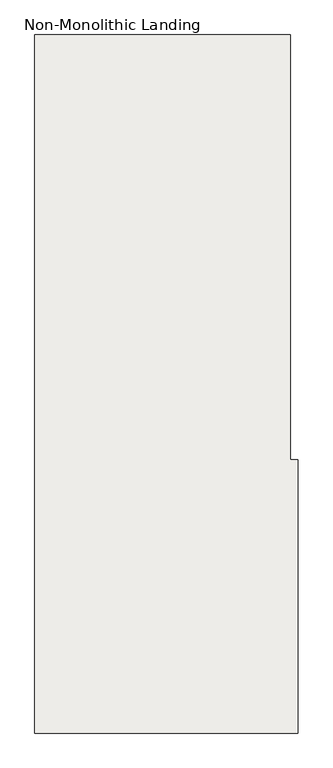
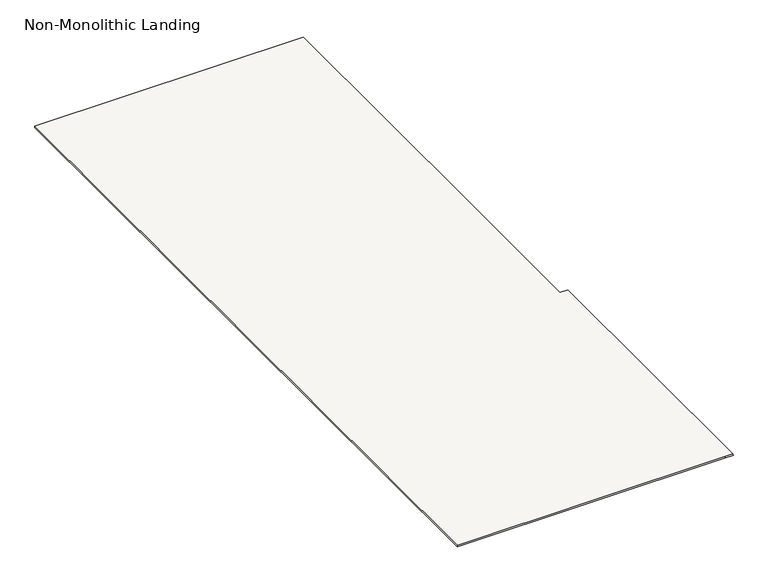
"""IFC4 building model written with IfcOpenShell, lengths in millimetres: slab geometry, Non-Monolithic Landing."""

from ifc_helpers import new_model, si_unit, origin, place, context, project, spatial, faceted_brep, source, transform, mapped, element, save


def non_monolithic_landing_7b62ab0d(model_context):
    return source(origin(), model_context, "Body", "Brep", [
        faceted_brep([(13356.0599092, 10220.4345331, 28470.5882353), (13356.9099092, 10220.4345331, 28464.5882353), (13356.9099092, 11395.4345331, 28464.5882353), (13356.0599092, 11395.4345331, 28470.5882353), (13325.0, 13220.4345331, 28470.5882353), (12225.0, 13220.4345331, 28470.5882353), (12225.0, 10220.4345331, 28470.5882353), (13325.0, 10220.4345331, 28470.5882353), (13325.0, 11395.4345331, 28470.5882353), (13325.0, 12030.4345331, 28470.5882353), (12225.0, 10220.4345331, 28464.5882353), (12225.0, 13220.4345331, 28464.5882353), (13324.15, 13220.4345331, 28464.5882353), (13324.15, 12030.4345331, 28464.5882353), (13325.0, 12030.4345331, 28464.5882353), (13325.0, 11395.4345331, 28464.5882353), (13325.0, 10220.4345331, 28464.5882353)], [[[0, 1, 2, 3]], [[4, 5, 6, 7, 0, 3, 8, 9]], [[10, 11, 12, 13, 14, 15, 2, 1, 16]], [[9, 8, 15, 14]], [[0, 7, 16, 1]], [[7, 6, 10, 16]], [[6, 5, 11, 10]], [[5, 4, 12, 11]], [[13, 9, 14]], [[9, 13, 12, 4]], [[8, 3, 2, 15]]]),
    ])


if __name__ == "__main__":
    model = new_model("IFC4")
    model_context = context("Model", 3, world=origin())
    ifc_project = project(units=[si_unit("LENGTHUNIT", "METRE", prefix="MILLI")], contexts=[model_context])
    site = spatial("IfcSite", under=ifc_project)
    building = spatial("IfcBuilding", under=site)
    placement = place(None, origin())
    non_monolithic_landing_shape = non_monolithic_landing_7b62ab0d(model_context)
    element("IfcSlab", 1, ObjectType="Non-Monolithic Landing", at=placement, inside=building, context=model_context, shape_type="MappedRepresentation", body=[
        mapped(non_monolithic_landing_shape, transform((0.0, 0.0, 0.0), x_axis=(1.0, 0.0, 0.0), y_axis=(0.0, 1.0, 0.0), z_axis=(0.0, 0.0, 1.0))),
    ])
    save(model, "model.ifc")

# Revit data of these elements
# Element 1 (IfcSlab, "Non-Monolithic Landing")
#   Materials on its faces: "Steel, Paint Finish, Dark Gray"
# Materials
#   "Steel, Paint Finish, Dark Gray": class "Metal", colour RGB 89 89 89, transparency 0, Description = "Steel, paint finish, dark gray, glossy", Cost = 0
